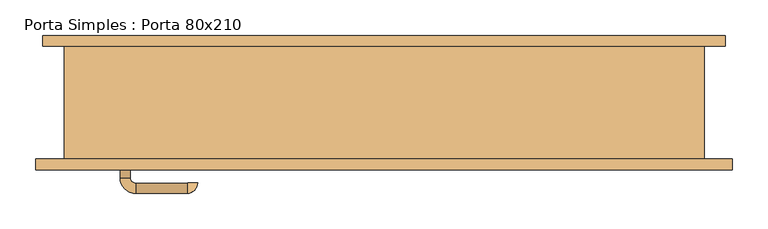
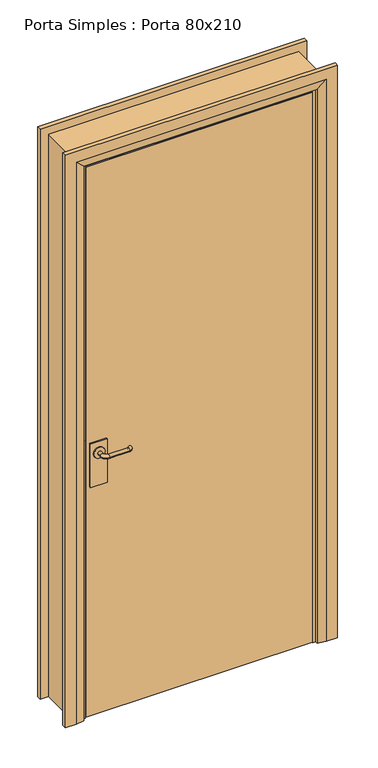
"""IFC4 building model written with IfcOpenShell, lengths in millimetres: door geometry, Porta Simples : Porta 80x210."""

import ifcopenshell
import ifcopenshell.guid

model = None  # the IFC model being written
_history = None  # IfcOwnerHistory: only IFC2X3 demands one
_inside = {}  # id of a spatial element -> (the spatial element, [elements in it])
_under = {}  # id of a project, library or spatial element -> (it, [spatial elements below it])
_declared = {}  # id of a project -> (the project, [libraries it declares])
_typed = {}  # id of a type object -> (the type object, [elements of that type])
_made_of = {}  # id of a material, layer set ... -> (it, [elements and type objects made of it])


def new_model(schema):
    """Start an empty IFC model of exactly this schema.

    Asked for "IFC4X3", IfcOpenShell would pick the latest addendum, in which some entities
    have other attributes; the version numbers below select the first issue.
    IFC2X3 requires an IfcOwnerHistory on every rooted entity: one is made here for all.
    """
    global model, _history
    if schema == "IFC4X3":
        model = ifcopenshell.file(schema_version=(4, 3, 0, 0))
    else:
        model = ifcopenshell.file(schema=schema)
    _inside.clear()
    _under.clear()
    _declared.clear()
    _typed.clear()
    _made_of.clear()
    _history = None
    if model.schema == "IFC2X3":
        org = make("IfcOrganization", Name="unknown")
        user = make(
            "IfcPersonAndOrganization",
            ThePerson=make("IfcPerson", FamilyName="unknown"),
            TheOrganization=org,
        )
        app = make(
            "IfcApplication",
            ApplicationDeveloper=org,
            Version="unknown",
            ApplicationFullName="unknown",
            ApplicationIdentifier="unknown",
        )
        _history = make(
            "IfcOwnerHistory",
            OwningUser=user,
            OwningApplication=app,
            ChangeAction="ADDED",
            CreationDate=0,
        )
    return model


def make(cls, **values):
    """One entity of the class cls with the attributes given. An attribute that is None is left unset."""
    return model.create_entity(
        cls, **{name: value for name, value in values.items() if value is not None}
    )


def rooted(cls, **values):
    """An entity with a GlobalId (a new one), such as an element, a storey or a relation."""
    return make(cls, GlobalId=ifcopenshell.guid.new(), OwnerHistory=_history, **values)


def si_unit(unit_type, name, prefix=None):
    """IfcSIUnit, for example si_unit("LENGTHUNIT", "METRE", prefix="MILLI")."""
    return make("IfcSIUnit", UnitType=unit_type, Prefix=prefix, Name=name)


def assignment(units):
    """IfcUnitAssignment: the units of a project."""
    return None if units is None else make("IfcUnitAssignment", Units=units)


def point(xyz):
    """IfcCartesianPoint."""
    return None if xyz is None else make("IfcCartesianPoint", Coordinates=xyz)


def direction(xyz):
    """IfcDirection."""
    return None if xyz is None else make("IfcDirection", DirectionRatios=xyz)


def frame(location, z_axis=None, x_axis=None):
    """IfcAxis2Placement3D, a coordinate frame: its origin and axes. An axis left out is left unset."""
    return make(
        "IfcAxis2Placement3D",
        Location=point(location),
        Axis=direction(z_axis),
        RefDirection=direction(x_axis),
    )


def frame_2d(location, x_axis=None):
    """IfcAxis2Placement2D, a coordinate frame in the plane: its origin and x axis."""
    return make(
        "IfcAxis2Placement2D", Location=point(location), RefDirection=direction(x_axis)
    )


def origin():
    """The frame at (0, 0, 0) with its axes left unset."""
    return frame((0.0, 0.0, 0.0))


def place(relative_to, where):
    """IfcLocalPlacement: puts the frame where relative to a parent placement (None: the world)."""
    return make(
        "IfcLocalPlacement", PlacementRelTo=relative_to, RelativePlacement=where
    )


def context(
    kind, dimensions, precision=None, world=None, true_north=None, identifier=None
):
    """IfcGeometricRepresentationContext, for example the 3D "Model" context."""
    return make(
        "IfcGeometricRepresentationContext",
        ContextIdentifier=identifier,
        ContextType=kind,
        CoordinateSpaceDimension=dimensions,
        Precision=precision,
        WorldCoordinateSystem=world,
        TrueNorth=true_north,
    )


def project(units=None, contexts=None):
    """IfcProject with its units and contexts."""
    return rooted(
        "IfcProject",
        Name="project",
        RepresentationContexts=contexts,
        UnitsInContext=assignment(units),
    )


def spatial(cls, under=None, at=None, **own):
    """A site, building, storey or space (cls), placed at a placement, below another one or the project."""
    s = rooted(cls, ObjectPlacement=at, **own)
    if under is not None:
        _under.setdefault(under.id(), (under, []))[1].append(s)
    return s


def polyline(points):
    """IfcPolyline through the points."""
    return make("IfcPolyline", Points=[point(p) for p in points])


def circle_curve(where, radius):
    """IfcCircle in the frame where."""
    return make("IfcCircle", Position=where, Radius=radius)


def ellipse_curve(where, semi_axis1, semi_axis2):
    """IfcEllipse in the frame where."""
    return make(
        "IfcEllipse", Position=where, SemiAxis1=semi_axis1, SemiAxis2=semi_axis2
    )


def trimmed(basis, trim1, trim2, sense, master):
    """IfcTrimmedCurve: the piece of a basis curve between two trims."""
    return make(
        "IfcTrimmedCurve",
        BasisCurve=basis,
        Trim1=trim1,
        Trim2=trim2,
        SenseAgreement=sense,
        MasterRepresentation=master,
    )


def segment(curve, same_sense, transition):
    """IfcCompositeCurveSegment."""
    return make(
        "IfcCompositeCurveSegment",
        Transition=transition,
        SameSense=same_sense,
        ParentCurve=curve,
    )


def composite_curve(segments, self_intersect=None):
    """IfcCompositeCurve: segments joined end to end."""
    return make("IfcCompositeCurve", Segments=segments, SelfIntersect=self_intersect)


def outline(outer, holes=None, kind="AREA"):
    """IfcArbitraryClosedProfileDef: a profile drawn as a closed curve; with holes, ...WithVoids."""
    if holes is None:
        return make("IfcArbitraryClosedProfileDef", ProfileType=kind, OuterCurve=outer)
    return make(
        "IfcArbitraryProfileDefWithVoids",
        ProfileType=kind,
        OuterCurve=outer,
        InnerCurves=holes,
    )


def extrude(swept, where, along, depth):
    """IfcExtrudedAreaSolid: the profile swept, set in the frame where, extruded along a direction by depth."""
    return make(
        "IfcExtrudedAreaSolid",
        SweptArea=swept,
        Position=where,
        ExtrudedDirection=direction(along),
        Depth=depth,
    )


def faces_of(points, faces, orient=None, outer=None):
    """IfcFace entities. A face is a list of loops; a loop is a list of indices into points, from 0.

    orient and outer hold one flag for each loop. By default every Orientation is true, the
    first loop of a face is its IfcFaceOuterBound and the others are IfcFaceBound.
    """
    made = []
    for i, loops in enumerate(faces):
        bounds = []
        for j, loop in enumerate(loops):
            is_outer = j == 0 if outer is None else outer[i][j]
            bounds.append(
                make(
                    "IfcFaceOuterBound" if is_outer else "IfcFaceBound",
                    Bound=make("IfcPolyLoop", Polygon=[points[k] for k in loop]),
                    Orientation=True if orient is None else orient[i][j],
                )
            )
        made.append(make("IfcFace", Bounds=bounds))
    return made


def faceted_brep(points, faces, orient=None, outer=None, voids=None):
    """IfcFacetedBrep: a solid bounded by flat faces; with voids (closed shells), ...WithVoids."""
    shared = [point(p) for p in points]
    hull = make("IfcClosedShell", CfsFaces=faces_of(shared, faces, orient, outer))
    if voids is None:
        return make("IfcFacetedBrep", Outer=hull)
    return make(
        "IfcFacetedBrepWithVoids",
        Outer=hull,
        Voids=[
            make(cls, CfsFaces=faces_of(shared, fs, o, b)) for cls, fs, o, b in voids
        ],
    )


def shape(context_of_items, identifier, shape_type, items):
    """IfcShapeRepresentation: the items that make up one representation, for example the "Body"."""
    return make(
        "IfcShapeRepresentation",
        ContextOfItems=context_of_items,
        RepresentationIdentifier=identifier,
        RepresentationType=shape_type,
        Items=items,
    )


def source(mapping_origin, context_of_items, identifier, shape_type, items):
    """IfcRepresentationMap: a shape defined once, which mapped items show again and again."""
    return make(
        "IfcRepresentationMap",
        MappingOrigin=mapping_origin,
        MappedRepresentation=shape(context_of_items, identifier, shape_type, items),
    )


def transform(
    local_origin,
    x_axis=None,
    y_axis=None,
    z_axis=None,
    scale=None,
    scale2=None,
    scale3=None,
    uniform=True,
):
    """IfcCartesianTransformationOperator3D, or its non-uniform kind. x_axis, y_axis, z_axis: its Axis1, 2, 3."""
    if uniform:
        return make(
            "IfcCartesianTransformationOperator3D",
            Axis1=direction(x_axis),
            Axis2=direction(y_axis),
            LocalOrigin=point(local_origin),
            Scale=scale,
            Axis3=direction(z_axis),
        )
    return make(
        "IfcCartesianTransformationOperator3DnonUniform",
        Axis1=direction(x_axis),
        Axis2=direction(y_axis),
        LocalOrigin=point(local_origin),
        Scale=scale,
        Axis3=direction(z_axis),
        Scale2=scale2,
        Scale3=scale3,
    )


def mapped(mapping_source, mapping_target):
    """IfcMappedItem: shows the shape of a source again, moved by a transform."""
    return make(
        "IfcMappedItem", MappingSource=mapping_source, MappingTarget=mapping_target
    )


def made_of(thing, what):
    """Note that an element or type object is made of a material, layer set ...; save() writes the relation."""
    if what is not None:
        _made_of.setdefault(what.id(), (what, []))[1].append(thing)
    return thing


def element(
    cls,
    number,
    at=None,
    inside=None,
    cuts=None,
    type_object=None,
    material=None,
    context=None,
    identifier="Body",
    shape_type=None,
    held_by="IfcProductDefinitionShape",
    body=None,
    shapes=None,
    **own,
):
    """One element of the class cls, such as IfcWall. Its Tag is "e" and its number.

    at: its placement. inside: the storey or other place that contains it. cuts: it is an
    opening in that element (IfcRelVoidsElement). A single representation is given by context,
    identifier, shape_type and body (its items); several are given by shapes. held_by: the class
    of the entity that holds the representations. save() writes the other relations.
    """
    e = rooted(cls, Tag="e%d" % number, ObjectPlacement=at, **own)
    if body is not None:
        shapes = [shape(context, identifier, shape_type, body)]
    if shapes is not None:
        e.Representation = make(held_by, Representations=shapes)
    if inside is not None:
        _inside.setdefault(inside.id(), (inside, []))[1].append(e)
    if cuts is not None:
        rooted(
            "IfcRelVoidsElement", RelatingBuildingElement=cuts, RelatedOpeningElement=e
        )
    if type_object is not None:
        _typed.setdefault(type_object.id(), (type_object, []))[1].append(e)
    return made_of(e, material)


def aggregate(whole, parts):
    """IfcRelAggregates: a whole, such as a stair, and the parts it consists of."""
    return rooted("IfcRelAggregates", RelatingObject=whole, RelatedObjects=parts)


def save(model, path):
    """Write the relations noted so far, then the file.

    IfcRelAggregates (storeys below a building ...), IfcRelContainedInSpatialStructure (elements
    in a storey), IfcRelDefinesByType, IfcRelAssociatesMaterial and IfcRelDeclares: one each for
    every whole, place, type object, material and project.
    """
    for whole, parts in _under.values():
        aggregate(whole, parts)
    for where, things in _inside.values():
        rooted(
            "IfcRelContainedInSpatialStructure",
            RelatedElements=things,
            RelatingStructure=where,
        )
    for kind, things in _typed.values():
        rooted("IfcRelDefinesByType", RelatedObjects=things, RelatingType=kind)
    for what, things in _made_of.values():
        rooted("IfcRelAssociatesMaterial", RelatedObjects=things, RelatingMaterial=what)
    for by, libraries in _declared.values():
        rooted("IfcRelDeclares", RelatingContext=by, RelatedDefinitions=libraries)
    model.write(path)


def plane_surface(at):
    """IfcPlane: the flat surface through the origin of the frame at, square to its z axis."""
    return make("IfcPlane", Position=at)


def cylinder_surface(at, radius):
    """IfcCylindricalSurface: all points at the distance radius from the z axis of the frame at."""
    return make("IfcCylindricalSurface", Position=at, Radius=radius)


def revolved_surface(curve, axis_point, axis_direction):
    """IfcSurfaceOfRevolution: the curve turned about the line through axis_point along axis_direction."""
    return make(
        "IfcSurfaceOfRevolution",
        SweptCurve=make("IfcArbitraryOpenProfileDef", ProfileType="CURVE", Curve=curve),
        AxisPosition=make("IfcAxis1Placement", Location=point(axis_point), Axis=direction(axis_direction)),
    )


def advanced_brep(points, edges, surfaces, faces):
    """IfcAdvancedBrep: a solid bounded by faces that lie on surfaces and meet in shared edges.

    An edge is (start, end): straight between two places in points (the first is 0);
    or (start, end, curve); or (start, end, curve, False) where it runs against its curve.
    A face is (place in surfaces, loops), or (place, loops, False) where it looks against
    its surface's normal. A loop lists edges by number (the first is 1), with a minus sign
    where the edge is run from its end to its start. The first loop is the outer one.
    """
    corners = [point(p) for p in points]
    vertices = [make("IfcVertexPoint", VertexGeometry=c) for c in corners]
    made = []
    for start, end, *more in edges:
        made.append(
            make(
                "IfcEdgeCurve",
                EdgeStart=vertices[start],
                EdgeEnd=vertices[end],
                EdgeGeometry=more[0] if more else make("IfcPolyline", Points=[corners[start], corners[end]]),
                SameSense=more[1] if len(more) > 1 else True,
            )
        )
    hull = []
    for where, loops, *sense in faces:
        bounds = []
        for j, loop in enumerate(loops):
            ring = [make("IfcOrientedEdge", EdgeElement=made[abs(k) - 1], Orientation=k > 0) for k in loop]
            bounds.append(
                make(
                    "IfcFaceOuterBound" if j == 0 else "IfcFaceBound",
                    Bound=make("IfcEdgeLoop", EdgeList=ring),
                    Orientation=True,
                )
            )
        hull.append(make("IfcAdvancedFace", Bounds=bounds, FaceSurface=surfaces[where], SameSense=sense[0] if sense else True))
    return make("IfcAdvancedBrep", Outer=make("IfcClosedShell", CfsFaces=hull))


def porta_simples_porta_80x210_1d639e12(model_context):
    return source(origin(), model_context, "Body", "SolidModel", [
        extrude(outline(composite_curve([segment(trimmed(circle_curve(frame_2d((1050.0, -364.0)), 20.0), [point((1050.0, -384.0))], [point((1050.0, -344.0))], False, "CARTESIAN"), True, "CONTINUOUS"), segment(trimmed(circle_curve(frame_2d((1050.0, -364.0)), 20.0), [point((1050.0, -344.0))], [point((1050.0, -384.0))], False, "CARTESIAN"), True, "CONTINUOUS")], self_intersect=False)), frame((0.0, -38.6, 0.0), z_axis=(0.0, 1.0, 0.0), x_axis=(0.0, 0.0, 1.0)), (0.0, 0.0, 1.0), 4.5929895),
        advanced_brep(
        [(-357.0, -34.0070105, 1050.0), (-371.0, -34.0070105, 1050.0), (-357.0, -18.6, 1050.0), (-371.0, -18.6, 1050.0), (-349.0, 3.4, 1050.0), (-349.0, -10.6, 1050.0), (-277.0, -10.6, 1050.0), (-277.0, 3.4, 1050.0), (-276.0, -11.6, 1050.0), (-262.0, -11.6, 1050.0)],
        [
            (0, 1, circle_curve(frame((-364.0, -34.0070105, 1050.0), z_axis=(0.0, -1.0, 0.0), x_axis=(-1.0, 0.0, 0.0)), 7.0)),
            (1, 0, circle_curve(frame((-364.0, -34.0070105, 1050.0), z_axis=(0.0, -1.0, 0.0), x_axis=(-1.0, 0.0, 0.0)), 7.0)),
            (0, 2),
            (2, 3, circle_curve(frame((-364.0, -18.6, 1050.0), z_axis=(0.0, -1.0, 0.0), x_axis=(-1.0, 0.0, 0.0)), 7.0)),
            (3, 1),
            (3, 2, circle_curve(frame((-364.0, -18.6, 1050.0), z_axis=(0.0, -1.0, 0.0), x_axis=(-1.0, 0.0, 0.0)), 7.0)),
            (4, 3, circle_curve(frame((-349.0, -18.6, 1050.0), z_axis=(0.0, 0.0, 1.0), x_axis=(-1.0, 0.0, 0.0)), 22.0)),
            (2, 5, circle_curve(frame((-349.0, -18.6, 1050.0), z_axis=(0.0, 0.0, -1.0), x_axis=(-1.0, 0.0, 0.0)), 8.0)),
            (5, 4, circle_curve(frame((-349.0, -3.6, 1050.0), z_axis=(-1.0, 0.0, 0.0), x_axis=(0.0, 1.0, 0.0)), 7.0)),
            (4, 5, circle_curve(frame((-349.0, -3.6, 1050.0), z_axis=(-1.0, 0.0, 0.0), x_axis=(0.0, 1.0, 0.0)), 7.0)),
            (5, 6),
            (6, 7, circle_curve(frame((-277.0, -3.6, 1050.0), z_axis=(-1.0, 0.0, 0.0), x_axis=(0.0, 1.0, 0.0)), 7.0)),
            (7, 4),
            (7, 6, circle_curve(frame((-277.0, -3.6, 1050.0), z_axis=(-1.0, 0.0, 0.0), x_axis=(0.0, 1.0, 0.0)), 7.0)),
            (8, 9, circle_curve(frame((-269.0, -11.6, 1050.0), z_axis=(0.0, -1.0, 0.0), x_axis=(1.0, 0.0, 0.0)), 7.0)),
            (9, 8, circle_curve(frame((-269.0, -11.6, 1050.0), z_axis=(0.0, -1.0, 0.0), x_axis=(1.0, 0.0, 0.0)), 7.0)),
            (9, 7, circle_curve(frame((-277.0, -11.6, 1050.0), z_axis=(0.0, 0.0, 1.0), x_axis=(0.0, 1.0, 0.0)), 15.0)),
            (6, 8, circle_curve(frame((-277.0, -11.6, 1050.0), z_axis=(0.0, 0.0, -1.0), x_axis=(0.0, 1.0, 0.0)), 1.0)),
        ],
        [
            plane_surface(frame((-364.0, -34.0070105, 1050.0), z_axis=(0.0, -1.0, 0.0), x_axis=(0.0, 0.0, 1.0))),
            cylinder_surface(frame((-364.0, -34.0070105, 1050.0), z_axis=(0.0, -1.0, 0.0), x_axis=(-1.0, 0.0, 0.0)), 7.0),
            revolved_surface(trimmed(ellipse_curve(frame((-364.0, -18.6, 1050.0), z_axis=(0.0, -1.0, 0.0), x_axis=(-1.0, 0.0, 0.0)), 7.0, 7.0), [point((-357.0, -18.6, 1050.0))], [point((-371.0, -18.6, 1050.0))], True, "CARTESIAN"), (-349.0, -18.6, 1050.0), (0.0, 0.0, -1.0)),
            revolved_surface(trimmed(ellipse_curve(frame((-364.0, -18.6, 1050.0), z_axis=(0.0, -1.0, 0.0), x_axis=(-1.0, 0.0, 0.0)), 7.0, 7.0), [point((-371.0, -18.6, 1050.0))], [point((-357.0, -18.6, 1050.0))], True, "CARTESIAN"), (-349.0, -18.6, 1050.0), (0.0, 0.0, -1.0)),
            cylinder_surface(frame((-349.0, -3.6, 1050.0), z_axis=(-1.0, 0.0, 0.0), x_axis=(0.0, 1.0, 0.0)), 7.0),
            plane_surface(frame((-269.0, -11.6, 1050.0), z_axis=(0.0, -1.0, 0.0), x_axis=(0.0, 0.0, 1.0))),
            revolved_surface(trimmed(ellipse_curve(frame((-277.0, -3.6, 1050.0), z_axis=(-1.0, 0.0, 0.0), x_axis=(0.0, 1.0, 0.0)), 7.0, 7.0), [point((-277.0, -10.6, 1050.0))], [point((-277.0, 3.4, 1050.0))], True, "CARTESIAN"), (-277.0, -11.6, 1050.0), (0.0, 0.0, -1.0)),
            revolved_surface(trimmed(ellipse_curve(frame((-277.0, -3.6, 1050.0), z_axis=(-1.0, 0.0, 0.0), x_axis=(0.0, 1.0, 0.0)), 7.0, 7.0), [point((-277.0, 3.4, 1050.0))], [point((-277.0, -10.6, 1050.0))], True, "CARTESIAN"), (-277.0, -11.6, 1050.0), (0.0, 0.0, -1.0)),
        ],
        [
            (0, [[1, 2]]),
            (1, [[-1, 3, 4, 5]]),
            (1, [[-2, -5, 6, -3]]),
            (2, [[7, -4, 8, 9]]),
            (3, [[-8, -6, -7, 10]]),
            (4, [[-9, 11, 12, 13]]),
            (4, [[-10, -13, 14, -11]]),
            (5, [[15, 16]]),
            (6, [[17, -12, 18, -16]]),
            (7, [[-18, -14, -17, -15]]),
        ],
    ),
        extrude(outline(polyline([(-334.0, -44.6), (-394.0, -44.6), (-394.0, -38.6), (-334.0, -38.6), (-334.0, -44.6)])), frame((0.0, 0.0, 925.0), z_axis=(0.0, 0.0, 1.0), x_axis=(1.0, 0.0, 0.0)), (0.0, 0.0, 1.0), 165.0),
        extrude(outline(composite_curve([segment(trimmed(circle_curve(frame_2d((1050.0, -364.0)), 20.0), [point((1050.0, -384.0))], [point((1050.0, -344.0))], False, "CARTESIAN"), True, "CONTINUOUS"), segment(trimmed(circle_curve(frame_2d((1050.0, -364.0)), 20.0), [point((1050.0, -344.0))], [point((1050.0, -384.0))], False, "CARTESIAN"), True, "CONTINUOUS")], self_intersect=False)), frame((0.0, -90.1929895, 0.0), z_axis=(0.0, 1.0, 0.0), x_axis=(0.0, 0.0, 1.0)), (0.0, 0.0, 1.0), 4.5929895),
        advanced_brep(
        [(-357.0, -90.1929895, 1050.0), (-371.0, -90.1929895, 1050.0), (-371.0, -105.6, 1050.0), (-357.0, -105.6, 1050.0), (-349.0, -127.6, 1050.0), (-349.0, -113.6, 1050.0), (-277.0, -127.6, 1050.0), (-277.0, -113.6, 1050.0), (-276.0, -112.6, 1050.0), (-262.0, -112.6, 1050.0)],
        [
            (0, 1, circle_curve(frame((-364.0, -90.1929895, 1050.0), z_axis=(0.0, 1.0, 0.0), x_axis=(-1.0, 0.0, 0.0)), 7.0)),
            (1, 0, circle_curve(frame((-364.0, -90.1929895, 1050.0), z_axis=(0.0, 1.0, 0.0), x_axis=(-1.0, 0.0, 0.0)), 7.0)),
            (1, 2),
            (2, 3, circle_curve(frame((-364.0, -105.6, 1050.0), z_axis=(0.0, 1.0, 0.0), x_axis=(-1.0, 0.0, 0.0)), 7.0)),
            (3, 0),
            (3, 2, circle_curve(frame((-364.0, -105.6, 1050.0), z_axis=(0.0, 1.0, 0.0), x_axis=(-1.0, 0.0, 0.0)), 7.0)),
            (4, 5, circle_curve(frame((-349.0, -120.6, 1050.0), z_axis=(-1.0, 0.0, 0.0), x_axis=(0.0, -1.0, 0.0)), 7.0)),
            (5, 3, circle_curve(frame((-349.0, -105.6, 1050.0), z_axis=(0.0, 0.0, -1.0), x_axis=(-1.0, 0.0, 0.0)), 8.0)),
            (2, 4, circle_curve(frame((-349.0, -105.6, 1050.0), z_axis=(0.0, 0.0, 1.0), x_axis=(-1.0, 0.0, 0.0)), 22.0)),
            (5, 4, circle_curve(frame((-349.0, -120.6, 1050.0), z_axis=(-1.0, 0.0, 0.0), x_axis=(0.0, -1.0, 0.0)), 7.0)),
            (4, 6),
            (6, 7, circle_curve(frame((-277.0, -120.6, 1050.0), z_axis=(-1.0, 0.0, 0.0), x_axis=(0.0, -1.0, 0.0)), 7.0)),
            (7, 5),
            (7, 6, circle_curve(frame((-277.0, -120.6, 1050.0), z_axis=(-1.0, 0.0, 0.0), x_axis=(0.0, -1.0, 0.0)), 7.0)),
            (8, 9, circle_curve(frame((-269.0, -112.6, 1050.0), z_axis=(0.0, 1.0, 0.0), x_axis=(1.0, 0.0, 0.0)), 7.0)),
            (9, 8, circle_curve(frame((-269.0, -112.6, 1050.0), z_axis=(0.0, 1.0, 0.0), x_axis=(1.0, 0.0, 0.0)), 7.0)),
            (8, 7, circle_curve(frame((-277.0, -112.6, 1050.0), z_axis=(0.0, 0.0, -1.0), x_axis=(0.0, -1.0, 0.0)), 1.0)),
            (6, 9, circle_curve(frame((-277.0, -112.6, 1050.0), z_axis=(0.0, 0.0, 1.0), x_axis=(0.0, -1.0, 0.0)), 15.0)),
        ],
        [
            plane_surface(frame((-364.0, -90.1929895, 1050.0), z_axis=(0.0, 1.0, 0.0), x_axis=(0.0, 0.0, 1.0))),
            cylinder_surface(frame((-364.0, -90.1929895, 1050.0), z_axis=(0.0, 1.0, 0.0), x_axis=(-1.0, 0.0, 0.0)), 7.0),
            revolved_surface(trimmed(ellipse_curve(frame((-364.0, -105.6, 1050.0), z_axis=(0.0, -1.0, 0.0), x_axis=(-1.0, 0.0, 0.0)), 7.0, 7.0), [point((-357.0, -105.6, 1050.0))], [point((-371.0, -105.6, 1050.0))], True, "CARTESIAN"), (-349.0, -105.6, 1050.0), (0.0, 0.0, -1.0)),
            revolved_surface(trimmed(ellipse_curve(frame((-364.0, -105.6, 1050.0), z_axis=(0.0, -1.0, 0.0), x_axis=(-1.0, 0.0, 0.0)), 7.0, 7.0), [point((-371.0, -105.6, 1050.0))], [point((-357.0, -105.6, 1050.0))], True, "CARTESIAN"), (-349.0, -105.6, 1050.0), (0.0, 0.0, -1.0)),
            cylinder_surface(frame((-349.0, -120.6, 1050.0), z_axis=(-1.0, 0.0, 0.0), x_axis=(0.0, -1.0, 0.0)), 7.0),
            plane_surface(frame((-269.0, -112.6, 1050.0), z_axis=(0.0, 1.0, 0.0), x_axis=(0.0, 0.0, 1.0))),
            revolved_surface(trimmed(ellipse_curve(frame((-277.0, -120.6, 1050.0), z_axis=(1.0, 0.0, 0.0), x_axis=(0.0, -1.0, 0.0)), 7.0, 7.0), [point((-277.0, -113.6, 1050.0))], [point((-277.0, -127.6, 1050.0))], True, "CARTESIAN"), (-277.0, -112.6, 1050.0), (0.0, 0.0, -1.0)),
            revolved_surface(trimmed(ellipse_curve(frame((-277.0, -120.6, 1050.0), z_axis=(1.0, 0.0, 0.0), x_axis=(0.0, -1.0, 0.0)), 7.0, 7.0), [point((-277.0, -127.6, 1050.0))], [point((-277.0, -113.6, 1050.0))], True, "CARTESIAN"), (-277.0, -112.6, 1050.0), (0.0, 0.0, -1.0)),
        ],
        [
            (0, [[1, 2]]),
            (1, [[3, 4, 5, -2]]),
            (1, [[-5, 6, -3, -1]]),
            (2, [[7, 8, -4, 9]]),
            (3, [[10, -9, -6, -8]]),
            (4, [[11, 12, 13, -7]]),
            (4, [[-13, 14, -11, -10]]),
            (5, [[15, 16]]),
            (6, [[-15, 17, -12, 18]]),
            (7, [[-16, -18, -14, -17]]),
        ],
    ),
        extrude(outline(polyline([(-334.0, -79.6), (-334.0, -85.6), (-394.0, -85.6), (-394.0, -79.6), (-334.0, -79.6)])), frame((0.0, 0.0, 925.0), z_axis=(0.0, 0.0, 1.0), x_axis=(1.0, 0.0, 0.0)), (0.0, 0.0, 1.0), 165.0),
        extrude(outline(polyline([(408.0, -44.6), (408.0, -79.6), (-408.0, -79.6), (-408.0, -44.6), (408.0, -44.6)])), frame((0.0, 0.0, 53.0), z_axis=(0.0, 0.0, 1.0), x_axis=(1.0, 0.0, 0.0)), (0.0, 0.0, 1.0), 2094.0),
        faceted_brep([(480.0, 79.6, 50.0), (410.0, 79.6, 50.0), (410.0, 89.6, 50.0), (440.0, 94.6, 50.0), (480.0, 94.6, 50.0), (480.0, 94.6, 2220.0), (480.0, 79.6, 2220.0), (440.0, 94.6, 2180.0), (-440.0, 94.6, 2180.0), (-440.0, 94.6, 50.0), (-480.0, 94.6, 50.0), (-480.0, 94.6, 2220.0), (410.0, 89.6, 2150.0), (410.0, 79.6, 2150.0), (-480.0, 79.6, 2220.0), (-480.0, 79.6, 50.0), (-410.0, 79.6, 50.0), (-410.0, 79.6, 2150.0), (-410.0, 89.6, 50.0), (-410.0, 89.6, 2150.0)], [[[0, 1, 2, 3, 4]], [[4, 5, 6, 0]], [[3, 7, 8, 9, 10, 11, 5, 4]], [[2, 12, 7, 3]], [[1, 13, 12, 2]], [[0, 6, 14, 15, 16, 17, 13, 1]], [[17, 16, 18, 19]], [[15, 10, 9, 18, 16]], [[11, 10, 15, 14]], [[19, 18, 9, 8]], [[13, 17, 19, 12]], [[5, 11, 14, 6]], [[12, 19, 8, 7]]]),
        faceted_brep([(490.0, -79.6, 50.0), (490.0, -94.6, 50.0), (450.0, -94.6, 50.0), (420.0, -89.6, 50.0), (420.0, -79.6, 50.0), (420.0, -79.6, 2160.0), (-420.0, -79.6, 2160.0), (-420.0, -79.6, 50.0), (-490.0, -79.6, 50.0), (-490.0, -79.6, 2230.0), (490.0, -79.6, 2230.0), (420.0, -89.6, 2160.0), (450.0, -94.6, 2190.0), (490.0, -94.6, 2230.0), (-490.0, -94.6, 2230.0), (-490.0, -94.6, 50.0), (-450.0, -94.6, 50.0), (-450.0, -94.6, 2190.0), (-420.0, -89.6, 50.0), (-420.0, -89.6, 2160.0)], [[[0, 1, 2, 3, 4]], [[4, 5, 6, 7, 8, 9, 10, 0]], [[3, 11, 5, 4]], [[2, 12, 11, 3]], [[1, 13, 14, 15, 16, 17, 12, 2]], [[0, 10, 13, 1]], [[9, 8, 15, 14]], [[8, 7, 18, 16, 15]], [[19, 18, 7, 6]], [[17, 16, 18, 19]], [[11, 19, 6, 5]], [[10, 9, 14, 13]], [[12, 17, 19, 11]]]),
        faceted_brep([(-410.0, -79.6, 50.0), (-450.0, -79.6, 50.0), (-450.0, 79.6, 50.0), (-400.0, 79.6, 50.0), (-400.0, -42.6, 50.0), (-410.0, -42.6, 50.0), (-410.0, -42.6, 2150.0), (-410.0, -79.6, 2150.0), (-400.0, -42.6, 2140.0), (-400.0, 79.6, 2140.0), (-450.0, 79.6, 2190.0), (-450.0, -79.6, 2190.0), (410.0, -79.6, 50.0), (410.0, -42.6, 50.0), (400.0, -42.6, 50.0), (400.0, 79.6, 50.0), (450.0, 79.6, 50.0), (450.0, -79.6, 50.0), (410.0, -79.6, 2150.0), (450.0, -79.6, 2190.0), (450.0, 79.6, 2190.0), (400.0, 79.6, 2140.0), (400.0, -42.6, 2140.0), (410.0, -42.6, 2150.0)], [[[0, 1, 2, 3, 4, 5]], [[5, 6, 7, 0]], [[4, 8, 6, 5]], [[3, 9, 8, 4]], [[2, 10, 9, 3]], [[1, 11, 10, 2]], [[0, 7, 11, 1]], [[12, 13, 14, 15, 16, 17]], [[18, 12, 17, 19]], [[19, 17, 16, 20]], [[20, 16, 15, 21]], [[21, 15, 14, 22]], [[22, 14, 13, 23]], [[23, 13, 12, 18]], [[6, 23, 18, 7]], [[8, 22, 23, 6]], [[9, 21, 22, 8]], [[10, 20, 21, 9]], [[11, 19, 20, 10]], [[7, 18, 19, 11]]]),
    ])


if __name__ == "__main__":
    model = new_model("IFC4")
    model_context = context("Model", 3, world=origin())
    ifc_project = project(units=[si_unit("LENGTHUNIT", "METRE", prefix="MILLI")], contexts=[model_context])
    site = spatial("IfcSite", under=ifc_project)
    building = spatial("IfcBuilding", under=site)
    placement = place(None, origin())
    porta_simples_porta_80x210_shape = porta_simples_porta_80x210_1d639e12(model_context)
    element("IfcDoor", 1, ObjectType="Porta Simples : Porta 80x210", at=placement, inside=building, context=model_context, shape_type="MappedRepresentation", body=[
        mapped(porta_simples_porta_80x210_shape, transform((0.0, 0.0, 0.0), x_axis=(1.0, 0.0, 0.0), y_axis=(0.0, 1.0, 0.0), z_axis=(0.0, 0.0, 1.0))),
    ])
    save(model, "model.ifc")

# Revit data of these elements
# Type "Porta Simples : Porta 80x210"
#   Type Mark = "49"
#   SINAPI = ""
#   Analytic Construction = "<Nenhum>"
#   Construction Type = "300"
#   Maçaneta [instance default] = ""
#   Fechadura [instance default] = ""
#   Vão Luz (somente para informação) = 0.78 m
#   Tolerância Folha Vertical = 0.003 m
#   Módulo Básico M = 0.10 m
#   Largura de Coordenação Modular Largura CM = 0.90 m
#   Rough Width = 0.90 m
#   Deslocamento da Horizontal da Folha = 0.00 m
#   Altura de Coordenação Modular Largura CM = 2.20 m
#   Rough Height = 2.20 m
#   Altura Nominal = 2.09 m
#   Ajuste de Coordenação Topo AC Topo = 0.01 m
#   Ajuste de Coordenação Base AC Base = 0.05 m
#   Ajuste de Coordenação AC = 0.01 m
#   Tolerância Folha Horizontal = 0.002 m
#   Largura Folha (somente para informação) = 0.796 m
#   Espessura Folha = 0.035 m
#   Maçaneta - Distância da Folha = 0.044 m
#   Maçaneta - Altura = 1.00 m
#   Largura Nominal (Largura Mn) = 0.82 m
#   Distância do Nível = 0.003 m
#   Aduela Interna Espessura = 0.04 m
#   Aduela Externa Espessura = 0.05 m
#   Altura Folha (somente para informação) = 2.075 m
#   Height = 2.14 m
#   Width = 0.88 m
#   Número de Módulos Básicos nM Largura = 9
#   Número de Módulos Básicos nM Altura = 22
#   Marco Metálico = no
#   Aduela de Madeira = no
#   Aduela Metálica de Canto = no
#   Guarnição Reta = no
#   Guarnição Chanfrada = yes
#   Batente - Material [instance default] = none
#   Painel - Material [instance default] = none
#   Model = ""
#   Function = (empty or 0)
#   Description = (empty or 0)
#   Wall Closure = (empty or 0)
#   Assembly Code = ""
# Element 1 (IfcDoor, "Porta Simples : Porta 80x210")
#   Materials on its faces: "Porta - Maçaneta"
# Materials
#   "Porta - Maçaneta": class "Diversos", colour RGB 0 0 0, transparency 0
